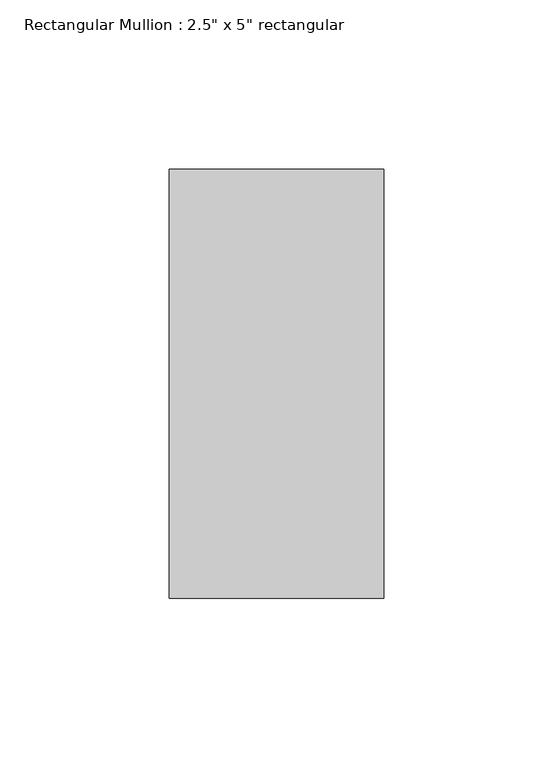
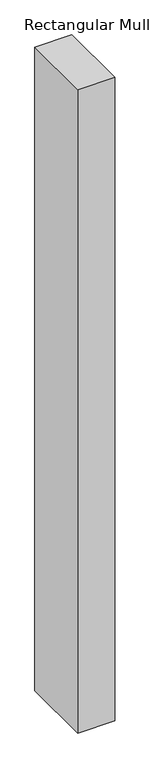
"""IFC4 building model written with IfcOpenShell, lengths in millimetres: member geometry."""

from ifc_helpers import new_model, si_unit, frame, origin, place, context, project, spatial, polyline, outline, extrude, source, transform, mapped, element, save


def member_f87cbf6c(model_context):
    return source(origin(), model_context, "Body", "SweptSolid", [
        extrude(outline(polyline([(31.75, 63.5), (31.75, -63.5), (-31.75, -63.5), (-31.75, 63.5), (31.75, 63.5)])), frame((0.0, 0.0, -1166.2833333), z_axis=(0.0, 0.0, 1.0), x_axis=(1.0, 0.0, 0.0)), (0.0, 0.0, 1.0), 1166.2833333),
    ])


if __name__ == "__main__":
    model = new_model("IFC4")
    model_context = context("Model", 3, world=origin())
    ifc_project = project(units=[si_unit("LENGTHUNIT", "METRE", prefix="MILLI")], contexts=[model_context])
    site = spatial("IfcSite", under=ifc_project)
    building = spatial("IfcBuilding", under=site)
    placement = place(None, origin())
    member_shape = member_f87cbf6c(model_context)
    element("IfcMember", 1, ObjectType="Rectangular Mullion : 2.5\" x 5\" rectangular", at=placement, inside=building, context=model_context, shape_type="MappedRepresentation", body=[
        mapped(member_shape, transform((0.0, 0.0, 0.0), x_axis=(1.0, 0.0, 0.0), y_axis=(0.0, 1.0, 0.0), z_axis=(0.0, 0.0, 1.0))),
    ])
    save(model, "model.ifc")

# Revit data of these elements
# Type "Rectangular Mullion : 2.5\" x 5\" rectangular"
#   built-in parameter 1007304 = 0.416667 (stored number, unit not read)
#   built-in parameter 1007301 = 0.104167 (stored number, unit not read)
#   built-in parameter 1007300 = 0.104167 (stored number, unit not read)
